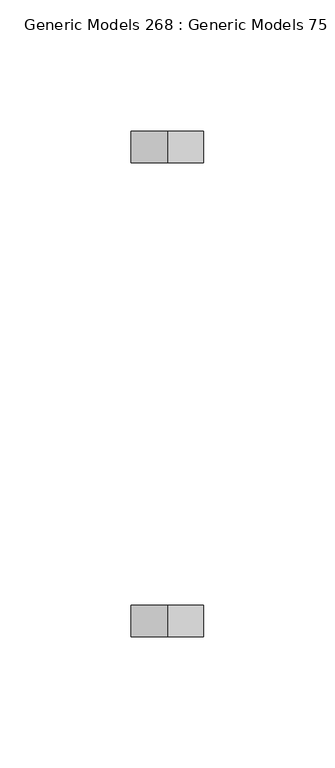
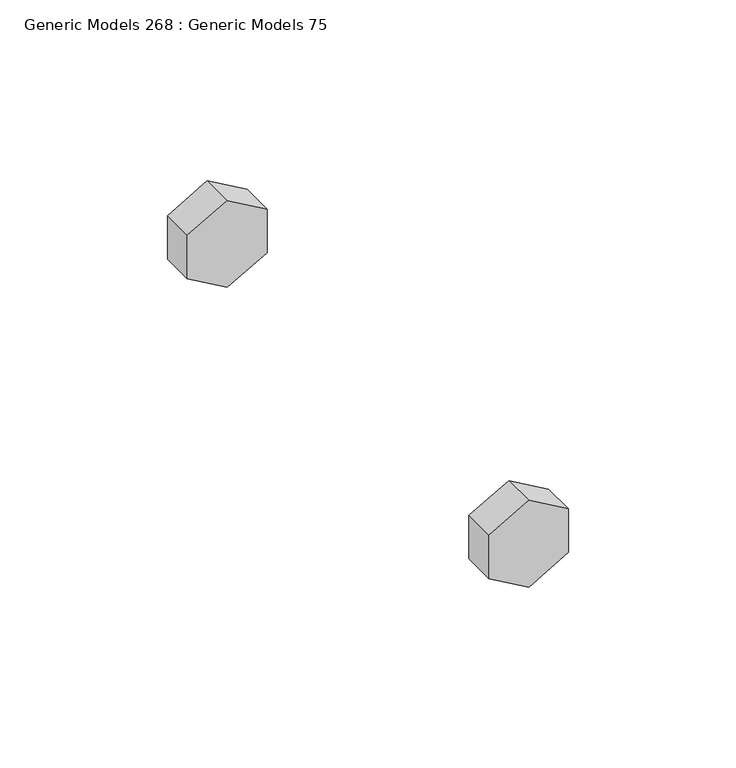
"""IFC4 building model written with IfcOpenShell, lengths in millimetres: proxy geometry, Generic Models 268 : Generic Models 75."""

from ifc_helpers import new_model, si_unit, frame, origin, place, context, project, spatial, polyline, outline, extrude, source, transform, mapped, element, save


def generic_models_268_generic_models_75_71ee5040(model_context):
    return source(origin(), model_context, "Body", "SweptSolid", [
        extrude(outline(polyline([(268613.0902933, 31975.9942029), (268597.2537198, 31975.9942029), (268589.335433, 31989.7090778), (268597.2537198, 32003.4239528), (268613.0902933, 32003.4239528), (268621.00858, 31989.7090778), (268613.0902933, 31975.9942029)])), frame((0.0, 30858.4781612, 0.0), z_axis=(0.0, 1.0, 0.0), x_axis=(0.0, 0.0, 1.0)), (0.0, 0.0, 1.0), 11.90625),
        extrude(outline(polyline([(268613.0902933, 31975.9942029), (268597.2537198, 31975.9942029), (268589.335433, 31989.7090778), (268597.2537198, 32003.4239528), (268613.0902933, 32003.4239528), (268621.00858, 31989.7090778), (268613.0902933, 31975.9942029)])), frame((0.0, 30678.2969112, 0.0), z_axis=(0.0, 1.0, 0.0), x_axis=(0.0, 0.0, 1.0)), (0.0, 0.0, 1.0), 11.90625),
    ])


if __name__ == "__main__":
    model = new_model("IFC4")
    model_context = context("Model", 3, world=origin())
    ifc_project = project(units=[si_unit("LENGTHUNIT", "METRE", prefix="MILLI")], contexts=[model_context])
    site = spatial("IfcSite", under=ifc_project)
    building = spatial("IfcBuilding", under=site)
    placement = place(None, origin())
    generic_models_268_generic_models_75_shape = generic_models_268_generic_models_75_71ee5040(model_context)
    element("IfcBuildingElementProxy", 1, Name="Generic Models 268 : Generic Models 75", ObjectType="Generic Models 268 : Generic Models 75", at=placement, inside=building, context=model_context, shape_type="MappedRepresentation", body=[
        mapped(generic_models_268_generic_models_75_shape, transform((0.0, 0.0, 0.0), x_axis=(1.0, 0.0, 0.0), y_axis=(0.0, 1.0, 0.0), z_axis=(0.0, 0.0, 1.0))),
    ])
    save(model, "model.ifc")

# Revit data of these elements
# Element 1 (IfcBuildingElementProxy, "Generic Models 268 : Generic Models 75")
#   Materials on its faces: "3/4\" GALV. THRU BOLTS"
# Materials
#   "3/4\" GALV. THRU BOLTS": class "Generic", colour RGB 105 69 171, transparency 0, Cost = 0
